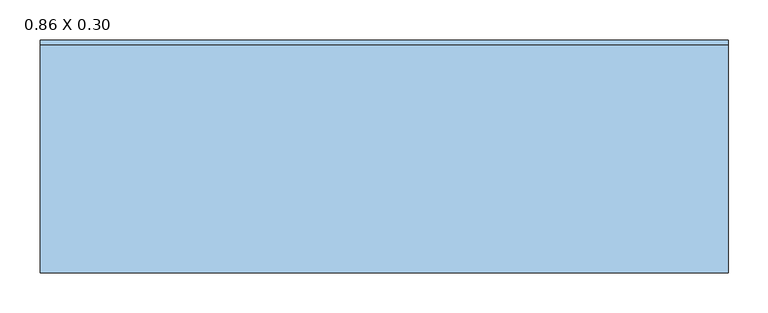
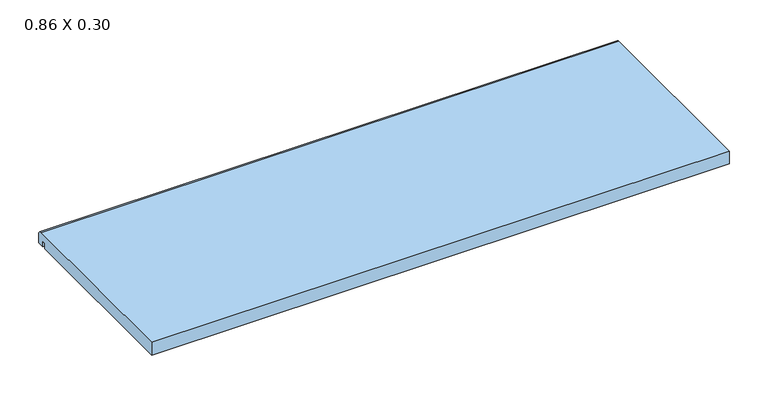
"""IFC4 building model written with IfcOpenShell, lengths in millimetres: window geometry, .CC_ND 300_PEDRA_PEITORIL RETO : 0.86 X 0.30."""

import ifcopenshell
import ifcopenshell.guid

model = None  # the IFC model being written
_history = None  # IfcOwnerHistory: only IFC2X3 demands one
_inside = {}  # id of a spatial element -> (the spatial element, [elements in it])
_under = {}  # id of a project, library or spatial element -> (it, [spatial elements below it])
_declared = {}  # id of a project -> (the project, [libraries it declares])
_typed = {}  # id of a type object -> (the type object, [elements of that type])
_made_of = {}  # id of a material, layer set ... -> (it, [elements and type objects made of it])


def new_model(schema):
    """Start an empty IFC model of exactly this schema.

    Asked for "IFC4X3", IfcOpenShell would pick the latest addendum, in which some entities
    have other attributes; the version numbers below select the first issue.
    IFC2X3 requires an IfcOwnerHistory on every rooted entity: one is made here for all.
    """
    global model, _history
    if schema == "IFC4X3":
        model = ifcopenshell.file(schema_version=(4, 3, 0, 0))
    else:
        model = ifcopenshell.file(schema=schema)
    _inside.clear()
    _under.clear()
    _declared.clear()
    _typed.clear()
    _made_of.clear()
    _history = None
    if model.schema == "IFC2X3":
        org = make("IfcOrganization", Name="unknown")
        user = make(
            "IfcPersonAndOrganization",
            ThePerson=make("IfcPerson", FamilyName="unknown"),
            TheOrganization=org,
        )
        app = make(
            "IfcApplication",
            ApplicationDeveloper=org,
            Version="unknown",
            ApplicationFullName="unknown",
            ApplicationIdentifier="unknown",
        )
        _history = make(
            "IfcOwnerHistory",
            OwningUser=user,
            OwningApplication=app,
            ChangeAction="ADDED",
            CreationDate=0,
        )
    return model


def make(cls, **values):
    """One entity of the class cls with the attributes given. An attribute that is None is left unset."""
    return model.create_entity(
        cls, **{name: value for name, value in values.items() if value is not None}
    )


def rooted(cls, **values):
    """An entity with a GlobalId (a new one), such as an element, a storey or a relation."""
    return make(cls, GlobalId=ifcopenshell.guid.new(), OwnerHistory=_history, **values)


def si_unit(unit_type, name, prefix=None):
    """IfcSIUnit, for example si_unit("LENGTHUNIT", "METRE", prefix="MILLI")."""
    return make("IfcSIUnit", UnitType=unit_type, Prefix=prefix, Name=name)


def assignment(units):
    """IfcUnitAssignment: the units of a project."""
    return None if units is None else make("IfcUnitAssignment", Units=units)


def point(xyz):
    """IfcCartesianPoint."""
    return None if xyz is None else make("IfcCartesianPoint", Coordinates=xyz)


def direction(xyz):
    """IfcDirection."""
    return None if xyz is None else make("IfcDirection", DirectionRatios=xyz)


def frame(location, z_axis=None, x_axis=None):
    """IfcAxis2Placement3D, a coordinate frame: its origin and axes. An axis left out is left unset."""
    return make(
        "IfcAxis2Placement3D",
        Location=point(location),
        Axis=direction(z_axis),
        RefDirection=direction(x_axis),
    )


def frame_2d(location, x_axis=None):
    """IfcAxis2Placement2D, a coordinate frame in the plane: its origin and x axis."""
    return make(
        "IfcAxis2Placement2D", Location=point(location), RefDirection=direction(x_axis)
    )


def origin():
    """The frame at (0, 0, 0) with its axes left unset."""
    return frame((0.0, 0.0, 0.0))


def place(relative_to, where):
    """IfcLocalPlacement: puts the frame where relative to a parent placement (None: the world)."""
    return make(
        "IfcLocalPlacement", PlacementRelTo=relative_to, RelativePlacement=where
    )


def context(
    kind, dimensions, precision=None, world=None, true_north=None, identifier=None
):
    """IfcGeometricRepresentationContext, for example the 3D "Model" context."""
    return make(
        "IfcGeometricRepresentationContext",
        ContextIdentifier=identifier,
        ContextType=kind,
        CoordinateSpaceDimension=dimensions,
        Precision=precision,
        WorldCoordinateSystem=world,
        TrueNorth=true_north,
    )


def project(units=None, contexts=None):
    """IfcProject with its units and contexts."""
    return rooted(
        "IfcProject",
        Name="project",
        RepresentationContexts=contexts,
        UnitsInContext=assignment(units),
    )


def spatial(cls, under=None, at=None, **own):
    """A site, building, storey or space (cls), placed at a placement, below another one or the project."""
    s = rooted(cls, ObjectPlacement=at, **own)
    if under is not None:
        _under.setdefault(under.id(), (under, []))[1].append(s)
    return s


def polyline(points):
    """IfcPolyline through the points."""
    return make("IfcPolyline", Points=[point(p) for p in points])


def circle_curve(where, radius):
    """IfcCircle in the frame where."""
    return make("IfcCircle", Position=where, Radius=radius)


def trimmed(basis, trim1, trim2, sense, master):
    """IfcTrimmedCurve: the piece of a basis curve between two trims."""
    return make(
        "IfcTrimmedCurve",
        BasisCurve=basis,
        Trim1=trim1,
        Trim2=trim2,
        SenseAgreement=sense,
        MasterRepresentation=master,
    )


def segment(curve, same_sense, transition):
    """IfcCompositeCurveSegment."""
    return make(
        "IfcCompositeCurveSegment",
        Transition=transition,
        SameSense=same_sense,
        ParentCurve=curve,
    )


def composite_curve(segments, self_intersect=None):
    """IfcCompositeCurve: segments joined end to end."""
    return make("IfcCompositeCurve", Segments=segments, SelfIntersect=self_intersect)


def outline(outer, holes=None, kind="AREA"):
    """IfcArbitraryClosedProfileDef: a profile drawn as a closed curve; with holes, ...WithVoids."""
    if holes is None:
        return make("IfcArbitraryClosedProfileDef", ProfileType=kind, OuterCurve=outer)
    return make(
        "IfcArbitraryProfileDefWithVoids",
        ProfileType=kind,
        OuterCurve=outer,
        InnerCurves=holes,
    )


def extrude(swept, where, along, depth):
    """IfcExtrudedAreaSolid: the profile swept, set in the frame where, extruded along a direction by depth."""
    return make(
        "IfcExtrudedAreaSolid",
        SweptArea=swept,
        Position=where,
        ExtrudedDirection=direction(along),
        Depth=depth,
    )


def shape(context_of_items, identifier, shape_type, items):
    """IfcShapeRepresentation: the items that make up one representation, for example the "Body"."""
    return make(
        "IfcShapeRepresentation",
        ContextOfItems=context_of_items,
        RepresentationIdentifier=identifier,
        RepresentationType=shape_type,
        Items=items,
    )


def source(mapping_origin, context_of_items, identifier, shape_type, items):
    """IfcRepresentationMap: a shape defined once, which mapped items show again and again."""
    return make(
        "IfcRepresentationMap",
        MappingOrigin=mapping_origin,
        MappedRepresentation=shape(context_of_items, identifier, shape_type, items),
    )


def transform(
    local_origin,
    x_axis=None,
    y_axis=None,
    z_axis=None,
    scale=None,
    scale2=None,
    scale3=None,
    uniform=True,
):
    """IfcCartesianTransformationOperator3D, or its non-uniform kind. x_axis, y_axis, z_axis: its Axis1, 2, 3."""
    if uniform:
        return make(
            "IfcCartesianTransformationOperator3D",
            Axis1=direction(x_axis),
            Axis2=direction(y_axis),
            LocalOrigin=point(local_origin),
            Scale=scale,
            Axis3=direction(z_axis),
        )
    return make(
        "IfcCartesianTransformationOperator3DnonUniform",
        Axis1=direction(x_axis),
        Axis2=direction(y_axis),
        LocalOrigin=point(local_origin),
        Scale=scale,
        Axis3=direction(z_axis),
        Scale2=scale2,
        Scale3=scale3,
    )


def mapped(mapping_source, mapping_target):
    """IfcMappedItem: shows the shape of a source again, moved by a transform."""
    return make(
        "IfcMappedItem", MappingSource=mapping_source, MappingTarget=mapping_target
    )


def made_of(thing, what):
    """Note that an element or type object is made of a material, layer set ...; save() writes the relation."""
    if what is not None:
        _made_of.setdefault(what.id(), (what, []))[1].append(thing)
    return thing


def element(
    cls,
    number,
    at=None,
    inside=None,
    cuts=None,
    type_object=None,
    material=None,
    context=None,
    identifier="Body",
    shape_type=None,
    held_by="IfcProductDefinitionShape",
    body=None,
    shapes=None,
    **own,
):
    """One element of the class cls, such as IfcWall. Its Tag is "e" and its number.

    at: its placement. inside: the storey or other place that contains it. cuts: it is an
    opening in that element (IfcRelVoidsElement). A single representation is given by context,
    identifier, shape_type and body (its items); several are given by shapes. held_by: the class
    of the entity that holds the representations. save() writes the other relations.
    """
    e = rooted(cls, Tag="e%d" % number, ObjectPlacement=at, **own)
    if body is not None:
        shapes = [shape(context, identifier, shape_type, body)]
    if shapes is not None:
        e.Representation = make(held_by, Representations=shapes)
    if inside is not None:
        _inside.setdefault(inside.id(), (inside, []))[1].append(e)
    if cuts is not None:
        rooted(
            "IfcRelVoidsElement", RelatingBuildingElement=cuts, RelatedOpeningElement=e
        )
    if type_object is not None:
        _typed.setdefault(type_object.id(), (type_object, []))[1].append(e)
    return made_of(e, material)


def aggregate(whole, parts):
    """IfcRelAggregates: a whole, such as a stair, and the parts it consists of."""
    return rooted("IfcRelAggregates", RelatingObject=whole, RelatedObjects=parts)


def save(model, path):
    """Write the relations noted so far, then the file.

    IfcRelAggregates (storeys below a building ...), IfcRelContainedInSpatialStructure (elements
    in a storey), IfcRelDefinesByType, IfcRelAssociatesMaterial and IfcRelDeclares: one each for
    every whole, place, type object, material and project.
    """
    for whole, parts in _under.values():
        aggregate(whole, parts)
    for where, things in _inside.values():
        rooted(
            "IfcRelContainedInSpatialStructure",
            RelatedElements=things,
            RelatingStructure=where,
        )
    for kind, things in _typed.values():
        rooted("IfcRelDefinesByType", RelatedObjects=things, RelatingType=kind)
    for what, things in _made_of.values():
        rooted("IfcRelAssociatesMaterial", RelatedObjects=things, RelatingMaterial=what)
    for by, libraries in _declared.values():
        rooted("IfcRelDeclares", RelatingContext=by, RelatedDefinitions=libraries)
    model.write(path)


def window_0_86_x_0_30_ebf489ac(model_context):
    return source(origin(), model_context, "Body", "SweptSolid", [
        extrude(outline(composite_curve([segment(polyline([(132.5083081, 1480.0), (-143.7, 1480.0), (-143.7, 1500.0), (141.3808343, 1500.0)]), True, "CONTINUOUS"), segment(trimmed(circle_curve(frame_2d((141.3808343, 1493.3808343)), 6.6191657), [point((141.3808343, 1500.0))], [point((148.0, 1493.3808343))], False, "CARTESIAN"), True, "CONTINUOUS"), segment(polyline([(148.0, 1493.3808343), (148.0, 1480.0), (137.2619526, 1480.0), (137.2619526, 1488.1993124), (132.5083081, 1488.1993124), (132.5083081, 1480.0)]), True, "CONTINUOUS")], self_intersect=False)), frame((-430.0, 0.0, 0.0), z_axis=(1.0, 0.0, 0.0), x_axis=(0.0, 1.0, 0.0)), (0.0, 0.0, 1.0), 860.0),
    ])


if __name__ == "__main__":
    model = new_model("IFC4")
    model_context = context("Model", 3, world=origin())
    ifc_project = project(units=[si_unit("LENGTHUNIT", "METRE", prefix="MILLI")], contexts=[model_context])
    site = spatial("IfcSite", under=ifc_project)
    building = spatial("IfcBuilding", under=site)
    placement = place(None, origin())
    window_0_86_x_0_30_shape = window_0_86_x_0_30_ebf489ac(model_context)
    element("IfcWindow", 1, ObjectType=".CC_ND 300_PEDRA_PEITORIL RETO : 0.86 X 0.30", at=placement, inside=building, context=model_context, shape_type="MappedRepresentation", body=[
        mapped(window_0_86_x_0_30_shape, transform((0.0, 0.0, 0.0), x_axis=(1.0, 0.0, 0.0), y_axis=(0.0, 1.0, 0.0), z_axis=(0.0, 0.0, 1.0))),
    ])
    save(model, "model.ifc")

# Revit data of these elements
# Type ".CC_ND 300_PEDRA_PEITORIL RETO : 0.86 X 0.30"
#   Type Mark = "66"
#   Largura da pedra [instance default] = 0.26 m
#   Extensão interior peitoril [instance default] = 0.03 m
#   Extensão exterior peitoril [instance default] = 0.03 m
#   Espessura = 0.02 m
#   Comprimento = 0.86 m
#   Altura-padrão do peitoril = 1.48 m
#   Peitoril = .GRANITO_BRANCO_ITAUNAS
#   Rough Width = 0
#   Rough Height = 0
#   Height = 0
#   Wall Closure = (empty or 0)
#   Width = 0
# Element 1 (IfcWindow, ".CC_ND 300_PEDRA_PEITORIL RETO : 0.86 X 0.30")
#   Largura da pedra = 0.2917 m
#   Extensão interior peitoril = 0.0257 m
#   Materials on its faces: ".GRANITO_BRANCO_ITAUNAS"
# Materials
#   ".GRANITO_BRANCO_ITAUNAS": class ".CC_PEDRA REVEST.", colour RGB 202 195 174, transparency 0, Description = "Revestimento em granito", Cost = 0
